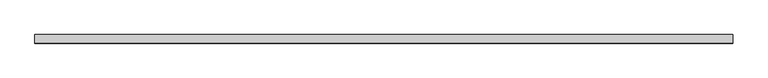
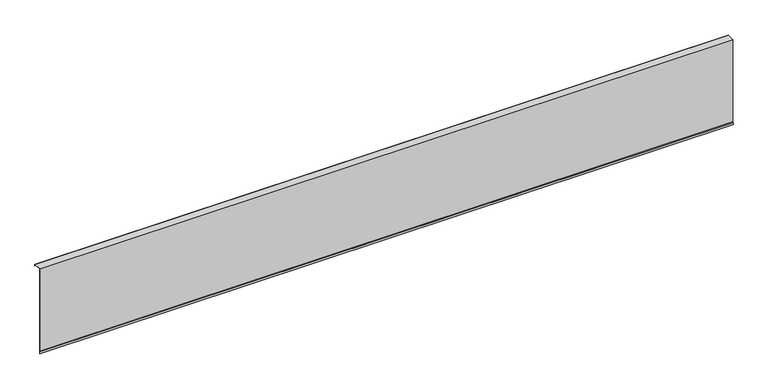
"""IFC4 building model written with IfcOpenShell, lengths in millimetres: proxy geometry, Generic Models 7:Generic Models 1:5:Generic Models 1:5 : Generic Models 7:Generic Models 1:337419:9 : Generic Models 7:Generic Models 1:5:Generic Models 1:5 : Generic Models 7:Generic Models 1:337419:311462."""

from ifc_helpers import new_model, si_unit, frame, origin, place, context, project, spatial, polyline, outline, extrude, source, transform, mapped, element, save


def generic_models_6faeec81(model_context):
    return source(origin(), model_context, "Body", "SweptSolid", [
        extrude(outline(polyline([(-579014.1851341, 3795.8885169), (-579025.7575229, 3779.361433), (-579025.7575229, 3725.3283058), (-579027.3450229, 3725.3283058), (-579027.3450229, 3779.8619698), (-579015.7726341, 3796.3890538), (-579015.7726341, 6180.6116872), (-578793.4990368, 6168.9628216), (-578793.4990368, 6125.115987), (-578795.0865368, 6125.115987), (-578795.0865368, 6167.4563403), (-579014.1851341, 6178.9388113), (-579014.1851341, 3795.8885169)])), frame((560352.1692831, 0.0, 0.0), z_axis=(1.0, 0.0, 0.0), x_axis=(0.0, 1.0, 0.0)), (0.0, 0.0, 1.0), 18970.6236908),
    ])


if __name__ == "__main__":
    model = new_model("IFC4")
    model_context = context("Model", 3, world=origin())
    ifc_project = project(units=[si_unit("LENGTHUNIT", "METRE", prefix="MILLI")], contexts=[model_context])
    site = spatial("IfcSite", under=ifc_project)
    building = spatial("IfcBuilding", under=site)
    placement = place(None, origin())
    generic_models_shape = generic_models_6faeec81(model_context)
    element("IfcBuildingElementProxy", 1, Name="Generic Models 7:Generic Models 1:5:Generic Models 1:5 : Generic Models 7:Generic Models 1:337419:9 : Generic Models 7:Generic Models 1:5:Generic Models 1:5 : Generic Models 7:Generic Models 1:337419:311462", ObjectType="Generic Models 7:Generic Models 1:5:Generic Models 1:5 : Generic Models 7:Generic Models 1:337419:9 : Generic Models 7:Generic Models 1:5:Generic Models 1:5 : Generic Models 7:Generic Models 1:337419:311462", at=placement, inside=building, context=model_context, shape_type="MappedRepresentation", body=[
        mapped(generic_models_shape, transform((0.0, 0.0, 0.0), x_axis=(1.0, 0.0, 0.0), y_axis=(0.0, 1.0, 0.0), z_axis=(0.0, 0.0, 1.0))),
    ])
    save(model, "model.ifc")

# Revit data of these elements
# Type "Generic Models 7:Generic Models 1:5:Generic Models 1:5 : Generic Models 7:Generic Models 1:337419:9 : Generic Models 7:Generic Models 1:5:Generic Models 1:5 : Generic Models 7:Generic Models 1:337419:311462"
#   NameOverride = "Generic Models 7:Generic Models 1:5:Generic Models 1:5 : Generic Models 7:Generic Models 1:337419:311462"
#   ObjectTypeOverride = "Generic Models 1:5 : Generic Models 7:Generic Models 1:337419"
#   Reference = "Generic Models 1"
#   Tag = "311462"
# Element 1 (IfcBuildingElementProxy, "Generic Models 7:Generic Models 1:5:Generic Models 1:5 : Generic Models 7:Generic Models 1:337419:9 : Generic Models 7:Generic Models 1:5:Generic Models 1:5 : Generic Models 7:Generic Models 1:337419:311462")
#   Materials on its faces: "UV STABLE WATER RESISTANT VAPOR PERMEABLE AIR BARRIER"
# Materials
#   "UV STABLE WATER RESISTANT VAPOR PERMEABLE AIR BARRIER": class "Generic", colour RGB 51 162 45, transparency 0, Description = "Polyethylene film membrane", Cost = 0
